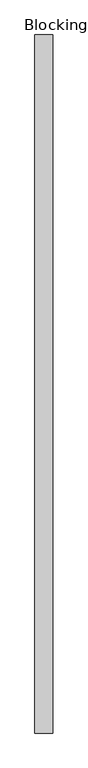
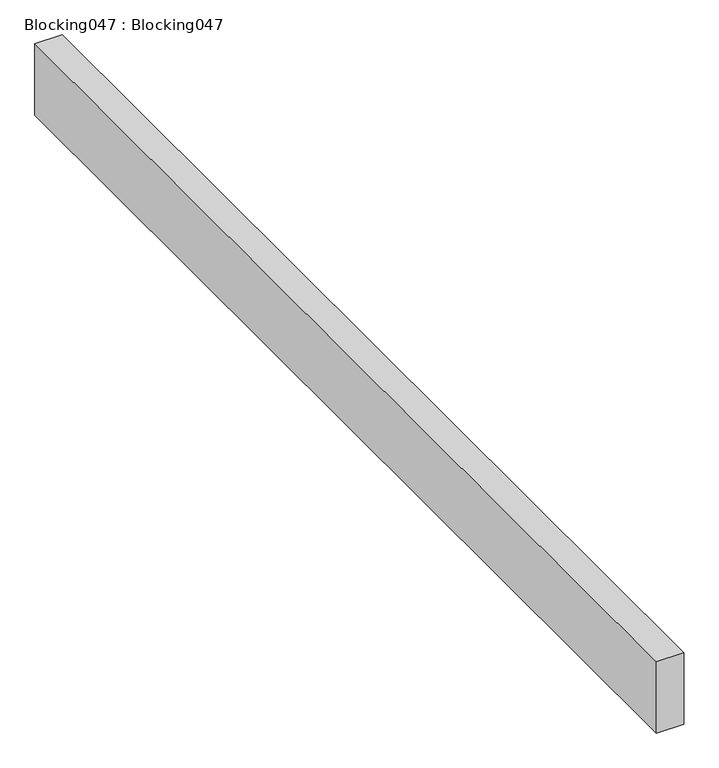
"""IFC4 building model written with IfcOpenShell, lengths in millimetres: proxy geometry, Blocking047 : Blocking047."""

import ifcopenshell
import ifcopenshell.guid

model = None  # the IFC model being written
_history = None  # IfcOwnerHistory: only IFC2X3 demands one
_inside = {}  # id of a spatial element -> (the spatial element, [elements in it])
_under = {}  # id of a project, library or spatial element -> (it, [spatial elements below it])
_declared = {}  # id of a project -> (the project, [libraries it declares])
_typed = {}  # id of a type object -> (the type object, [elements of that type])
_made_of = {}  # id of a material, layer set ... -> (it, [elements and type objects made of it])


def new_model(schema):
    """Start an empty IFC model of exactly this schema.

    Asked for "IFC4X3", IfcOpenShell would pick the latest addendum, in which some entities
    have other attributes; the version numbers below select the first issue.
    IFC2X3 requires an IfcOwnerHistory on every rooted entity: one is made here for all.
    """
    global model, _history
    if schema == "IFC4X3":
        model = ifcopenshell.file(schema_version=(4, 3, 0, 0))
    else:
        model = ifcopenshell.file(schema=schema)
    _inside.clear()
    _under.clear()
    _declared.clear()
    _typed.clear()
    _made_of.clear()
    _history = None
    if model.schema == "IFC2X3":
        org = make("IfcOrganization", Name="unknown")
        user = make(
            "IfcPersonAndOrganization",
            ThePerson=make("IfcPerson", FamilyName="unknown"),
            TheOrganization=org,
        )
        app = make(
            "IfcApplication",
            ApplicationDeveloper=org,
            Version="unknown",
            ApplicationFullName="unknown",
            ApplicationIdentifier="unknown",
        )
        _history = make(
            "IfcOwnerHistory",
            OwningUser=user,
            OwningApplication=app,
            ChangeAction="ADDED",
            CreationDate=0,
        )
    return model


def make(cls, **values):
    """One entity of the class cls with the attributes given. An attribute that is None is left unset."""
    return model.create_entity(
        cls, **{name: value for name, value in values.items() if value is not None}
    )


def rooted(cls, **values):
    """An entity with a GlobalId (a new one), such as an element, a storey or a relation."""
    return make(cls, GlobalId=ifcopenshell.guid.new(), OwnerHistory=_history, **values)


def si_unit(unit_type, name, prefix=None):
    """IfcSIUnit, for example si_unit("LENGTHUNIT", "METRE", prefix="MILLI")."""
    return make("IfcSIUnit", UnitType=unit_type, Prefix=prefix, Name=name)


def assignment(units):
    """IfcUnitAssignment: the units of a project."""
    return None if units is None else make("IfcUnitAssignment", Units=units)


def point(xyz):
    """IfcCartesianPoint."""
    return None if xyz is None else make("IfcCartesianPoint", Coordinates=xyz)


def direction(xyz):
    """IfcDirection."""
    return None if xyz is None else make("IfcDirection", DirectionRatios=xyz)


def frame(location, z_axis=None, x_axis=None):
    """IfcAxis2Placement3D, a coordinate frame: its origin and axes. An axis left out is left unset."""
    return make(
        "IfcAxis2Placement3D",
        Location=point(location),
        Axis=direction(z_axis),
        RefDirection=direction(x_axis),
    )


def origin():
    """The frame at (0, 0, 0) with its axes left unset."""
    return frame((0.0, 0.0, 0.0))


def place(relative_to, where):
    """IfcLocalPlacement: puts the frame where relative to a parent placement (None: the world)."""
    return make(
        "IfcLocalPlacement", PlacementRelTo=relative_to, RelativePlacement=where
    )


def context(
    kind, dimensions, precision=None, world=None, true_north=None, identifier=None
):
    """IfcGeometricRepresentationContext, for example the 3D "Model" context."""
    return make(
        "IfcGeometricRepresentationContext",
        ContextIdentifier=identifier,
        ContextType=kind,
        CoordinateSpaceDimension=dimensions,
        Precision=precision,
        WorldCoordinateSystem=world,
        TrueNorth=true_north,
    )


def project(units=None, contexts=None):
    """IfcProject with its units and contexts."""
    return rooted(
        "IfcProject",
        Name="project",
        RepresentationContexts=contexts,
        UnitsInContext=assignment(units),
    )


def spatial(cls, under=None, at=None, **own):
    """A site, building, storey or space (cls), placed at a placement, below another one or the project."""
    s = rooted(cls, ObjectPlacement=at, **own)
    if under is not None:
        _under.setdefault(under.id(), (under, []))[1].append(s)
    return s


def polyline(points):
    """IfcPolyline through the points."""
    return make("IfcPolyline", Points=[point(p) for p in points])


def outline(outer, holes=None, kind="AREA"):
    """IfcArbitraryClosedProfileDef: a profile drawn as a closed curve; with holes, ...WithVoids."""
    if holes is None:
        return make("IfcArbitraryClosedProfileDef", ProfileType=kind, OuterCurve=outer)
    return make(
        "IfcArbitraryProfileDefWithVoids",
        ProfileType=kind,
        OuterCurve=outer,
        InnerCurves=holes,
    )


def extrude(swept, where, along, depth):
    """IfcExtrudedAreaSolid: the profile swept, set in the frame where, extruded along a direction by depth."""
    return make(
        "IfcExtrudedAreaSolid",
        SweptArea=swept,
        Position=where,
        ExtrudedDirection=direction(along),
        Depth=depth,
    )


def shape(context_of_items, identifier, shape_type, items):
    """IfcShapeRepresentation: the items that make up one representation, for example the "Body"."""
    return make(
        "IfcShapeRepresentation",
        ContextOfItems=context_of_items,
        RepresentationIdentifier=identifier,
        RepresentationType=shape_type,
        Items=items,
    )


def source(mapping_origin, context_of_items, identifier, shape_type, items):
    """IfcRepresentationMap: a shape defined once, which mapped items show again and again."""
    return make(
        "IfcRepresentationMap",
        MappingOrigin=mapping_origin,
        MappedRepresentation=shape(context_of_items, identifier, shape_type, items),
    )


def transform(
    local_origin,
    x_axis=None,
    y_axis=None,
    z_axis=None,
    scale=None,
    scale2=None,
    scale3=None,
    uniform=True,
):
    """IfcCartesianTransformationOperator3D, or its non-uniform kind. x_axis, y_axis, z_axis: its Axis1, 2, 3."""
    if uniform:
        return make(
            "IfcCartesianTransformationOperator3D",
            Axis1=direction(x_axis),
            Axis2=direction(y_axis),
            LocalOrigin=point(local_origin),
            Scale=scale,
            Axis3=direction(z_axis),
        )
    return make(
        "IfcCartesianTransformationOperator3DnonUniform",
        Axis1=direction(x_axis),
        Axis2=direction(y_axis),
        LocalOrigin=point(local_origin),
        Scale=scale,
        Axis3=direction(z_axis),
        Scale2=scale2,
        Scale3=scale3,
    )


def mapped(mapping_source, mapping_target):
    """IfcMappedItem: shows the shape of a source again, moved by a transform."""
    return make(
        "IfcMappedItem", MappingSource=mapping_source, MappingTarget=mapping_target
    )


def made_of(thing, what):
    """Note that an element or type object is made of a material, layer set ...; save() writes the relation."""
    if what is not None:
        _made_of.setdefault(what.id(), (what, []))[1].append(thing)
    return thing


def element(
    cls,
    number,
    at=None,
    inside=None,
    cuts=None,
    type_object=None,
    material=None,
    context=None,
    identifier="Body",
    shape_type=None,
    held_by="IfcProductDefinitionShape",
    body=None,
    shapes=None,
    **own,
):
    """One element of the class cls, such as IfcWall. Its Tag is "e" and its number.

    at: its placement. inside: the storey or other place that contains it. cuts: it is an
    opening in that element (IfcRelVoidsElement). A single representation is given by context,
    identifier, shape_type and body (its items); several are given by shapes. held_by: the class
    of the entity that holds the representations. save() writes the other relations.
    """
    e = rooted(cls, Tag="e%d" % number, ObjectPlacement=at, **own)
    if body is not None:
        shapes = [shape(context, identifier, shape_type, body)]
    if shapes is not None:
        e.Representation = make(held_by, Representations=shapes)
    if inside is not None:
        _inside.setdefault(inside.id(), (inside, []))[1].append(e)
    if cuts is not None:
        rooted(
            "IfcRelVoidsElement", RelatingBuildingElement=cuts, RelatedOpeningElement=e
        )
    if type_object is not None:
        _typed.setdefault(type_object.id(), (type_object, []))[1].append(e)
    return made_of(e, material)


def aggregate(whole, parts):
    """IfcRelAggregates: a whole, such as a stair, and the parts it consists of."""
    return rooted("IfcRelAggregates", RelatingObject=whole, RelatedObjects=parts)


def save(model, path):
    """Write the relations noted so far, then the file.

    IfcRelAggregates (storeys below a building ...), IfcRelContainedInSpatialStructure (elements
    in a storey), IfcRelDefinesByType, IfcRelAssociatesMaterial and IfcRelDeclares: one each for
    every whole, place, type object, material and project.
    """
    for whole, parts in _under.values():
        aggregate(whole, parts)
    for where, things in _inside.values():
        rooted(
            "IfcRelContainedInSpatialStructure",
            RelatedElements=things,
            RelatingStructure=where,
        )
    for kind, things in _typed.values():
        rooted("IfcRelDefinesByType", RelatedObjects=things, RelatingType=kind)
    for what, things in _made_of.values():
        rooted("IfcRelAssociatesMaterial", RelatedObjects=things, RelatingMaterial=what)
    for by, libraries in _declared.values():
        rooted("IfcRelDeclares", RelatingContext=by, RelatedDefinitions=libraries)
    model.write(path)


def blocking047_blocking047_b324cb1b(model_context):
    return source(origin(), model_context, "Body", "SweptSolid", [
        extrude(outline(polyline([(-668.0864422, -1052.8908936), (-718.8864422, -1052.8908936), (-718.8864422, 947.1091064), (-668.0864422, 947.1091064), (-668.0864422, -1052.8908936)])), frame((0.0, 0.0, 39579.2960083), z_axis=(0.0, 0.0, 1.0), x_axis=(1.0, 0.0, 0.0)), (0.0, 0.0, 1.0), 139.7),
    ])


if __name__ == "__main__":
    model = new_model("IFC4")
    model_context = context("Model", 3, world=origin())
    ifc_project = project(units=[si_unit("LENGTHUNIT", "METRE", prefix="MILLI")], contexts=[model_context])
    site = spatial("IfcSite", under=ifc_project)
    building = spatial("IfcBuilding", under=site)
    placement = place(None, origin())
    blocking047_blocking047_shape = blocking047_blocking047_b324cb1b(model_context)
    element("IfcBuildingElementProxy", 1, Name="Blocking047 : Blocking047", ObjectType="Blocking047 : Blocking047", at=placement, inside=building, context=model_context, shape_type="MappedRepresentation", body=[
        mapped(blocking047_blocking047_shape, transform((0.0, 0.0, 0.0), x_axis=(1.0, 0.0, 0.0), y_axis=(0.0, 1.0, 0.0), z_axis=(0.0, 0.0, 1.0))),
    ])
    save(model, "model.ifc")

# Revit data of these elements
# Type "Blocking047 : Blocking047"
#   NameOverride = "Blocking047"
# Element 1 (IfcBuildingElementProxy, "Blocking047 : Blocking047")
#   Materials on its faces: "WOOD BLOCKING AS REQUIRED"
# Materials
#   "WOOD BLOCKING AS REQUIRED": class "Unassigned", colour RGB 166 124 85, transparency 0, Cost = 0
